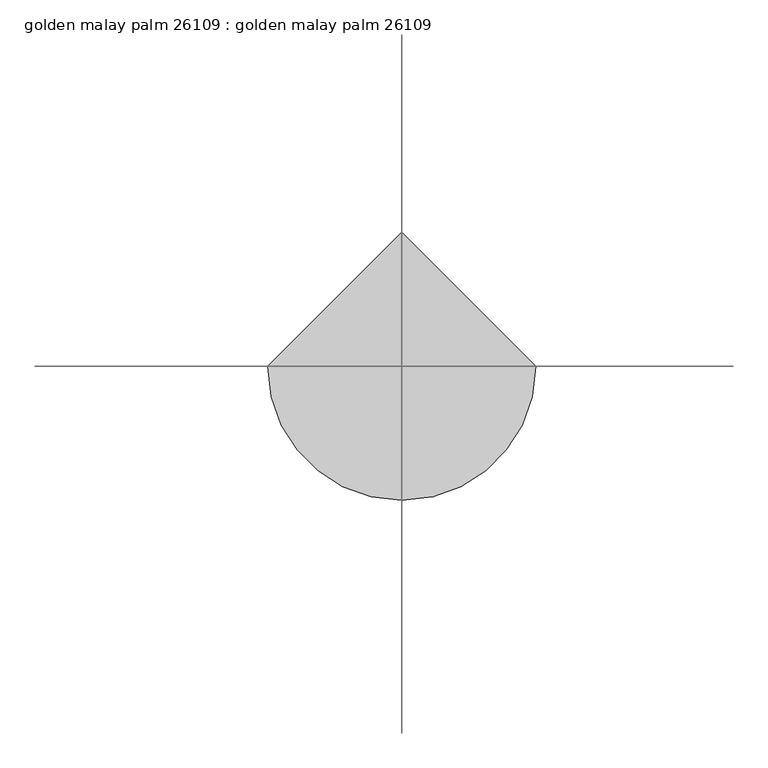
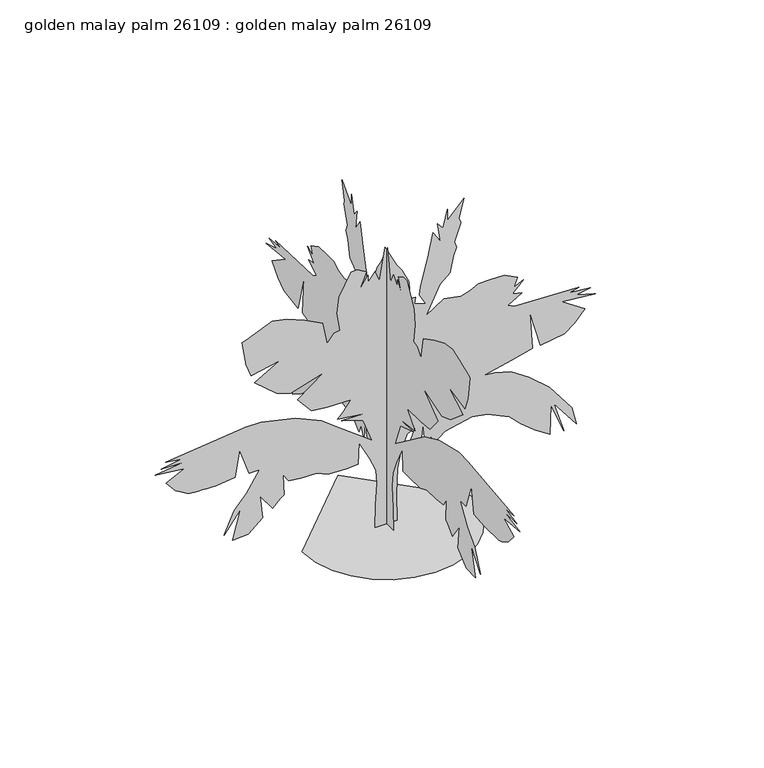
"""IFC4 building model written with IfcOpenShell, lengths in millimetres: proxy geometry, golden malay palm 26109 : golden malay palm 26109."""

from ifc_helpers import new_model, si_unit, origin, place, context, project, spatial, triangles, source, transform, mapped, element, save


def golden_malay_palm_26109_golden_malay_palm_26109_a310d7cf(model_context):
    return source(origin(), model_context, "Body", "Tessellation", [
        triangles([(9.89e-05, 133.5213922, 670.0644053), (0.0001158, 103.2936315, 529.0005229), (0.0001458, 93.2174569, 277.101182), (0.0001788, 98.2555397, 0.010878), (0.0001788, -113.3400931, 0.010878), (0.0001518, -108.30251, 226.7208087), (0.000126, -93.1884979, 443.3542972), (0.0001098, -103.2644181, 579.3813867), (9.23e-05, -163.7202029, 725.4820982), (6.95e-05, -264.479932, 916.9269533), (9.53e-05, -274.5561157, 700.292938), (9.59e-05, -385.3915197, 695.2536381), (9.53e-05, -561.7207641, 700.292938), (8.93e-05, -672.5587297, 750.671331), (8.93e-05, -828.7356068, 750.671331), (8.75e-05, -944.6103653, 765.7868328), (7.79e-05, -994.9887583, 846.3936859), (0.0001026, -984.9125565, 639.8358725), (0.0001056, -1025.2172184, 614.6467123), (0.0001146, -1095.7504858, 539.0766884), (9.47e-05, -1216.6620735, 705.3297672), (0.0001218, -1191.4703699, 478.6196228), (0.0001362, -1332.536832, 357.7080714), (0.0001368, -1483.6744091, 352.6712422), (0.0001026, -1403.067556, 639.8358725), (0.0001272, -1564.283733, 433.2780953), (0.000102, -1468.5613781, 644.8752451), (8.57e-05, -1347.6498631, 780.8998638), (6.23e-05, -1221.69883, 977.3814754), (6.23e-05, -1322.4607029, 977.3814754), (3.11e-05, -1413.1436852, 1239.3569092), (6.17e-05, -1458.4852489, 982.4207754), (6.41e-05, -1639.8538296, 962.2684444), (6.4e-05, -1687.1180958, 963.3555874), (6.38e-05, -1732.9753258, 964.4858963), (6.37e-05, -1776.0104897, 965.7050806), (6.35e-05, -1814.8165512, 967.0563789), (6.34e-05, -1847.9838581, 968.5828846), (6.32e-05, -1874.0976711, 970.3329231), (6.29e-05, -1891.7531342, 972.3446463), (6.24e-05, -1906.0304604, 976.2663546), (6.16e-05, -1922.6852577, 983.3606163), (6.04e-05, -1941.3262711, 993.0989754), (5.9e-05, -1961.5497459, 1004.9505775), (5.74e-05, -1982.9670433, 1018.3922716), (5.57e-05, -2005.1742634, 1032.8880438), (5.39e-05, -2027.7802963, 1047.9146702), (4.13e-05, -2118.4632786, 1153.7132269), (3.11e-05, -1947.1708271, 1239.3569092), (2.75e-05, -2224.261908, 1269.585442), (2.27e-05, -1952.2101997, 1309.8901039), (2.21e-05, -2168.844215, 1314.9270058), (1.79e-05, -1977.3993599, 1350.1949112), (1.55e-05, -2123.5001804, 1370.3471695), (5.3e-06, -1357.7259922, 1455.9909245), (5.3e-06, -1206.5858717, 1455.9909245), (1.43e-05, -874.0771706, 1380.4208279), (2.81e-05, -627.2171659, 1264.5486855), (4.37e-05, -455.9247508, 1133.5608959), (7.19e-05, -138.5302706, 896.7745497), (4.37e-05, -229.2143339, 1133.5608959), (3.59e-05, -435.7723835, 1199.0547907), (3.65e-05, -219.1381502, 1194.0154181), (3.23e-05, -471.0377455, 1229.2832508), (2.63e-05, -420.6568454, 1279.6617165), (1.43e-05, -340.0499923, 1380.4208279), (1.37e-05, -571.7995093, 1385.4602005), (1.19e-05, -722.9370501, 1400.5732315), (-7.4e-06, -858.9641396, 1561.7895538), (-2.96e-05, -607.064835, 1748.194891), (-1.82e-05, -924.4580343, 1652.4750069), (-2.36e-05, -1060.4851238, 1697.8165707), (-4.52e-05, -1272.0797665, 1879.1826805), (-6.14e-05, -1030.256591, 2015.2098427), (-5.48e-05, -1302.3082993, 1959.7921497), (-7.04e-05, -1352.6890903, 2090.7797939), (-9.86e-05, -1387.954525, 2327.5662128), (-9.98e-05, -1352.6890903, 2337.642342), (-0.000107, -1211.6227009, 2398.0967915), (-0.0001125, -1100.787315, 2443.4383553), (-0.0001095, -964.7627689, 2418.2491951), (-0.0001004, -788.4309448, 2342.6790985), (-8.96e-05, -617.1410368, 2251.9961163), (-6.32e-05, -571.7995093, 2030.3227283), (-7.28e-05, -506.3030711, 2110.9321976), (-7.4e-05, -445.848549, 2121.0083267), (-9.62e-05, -476.0770818, 2307.4138092), (-0.0001149, -455.9247508, 2463.5906136), (-0.0001401, -340.0499923, 2675.1776985), (-0.0001407, -284.6322812, 2680.2323318), (-0.0001347, -193.9479727, 2629.8386055), (-0.0001155, -259.443121, 2468.6301315), (-0.0001299, -178.834215, 2589.5288567), (-0.0001215, -178.834215, 2519.0084518), (-0.0001311, -113.3400931, 2599.6128342), (-0.0001185, -67.9985656, 2493.8192917), (-0.0001569, -17.6182708, 2816.2493202), (-0.0001311, 93.2174569, 2599.6128342), (-0.0001221, 148.6356586, 2524.0476791), (-0.0001052, 214.1292808, 2382.9839058), (-8.42e-05, 224.2057188, 2206.6545525), (-8.42e-05, 279.6234118, 2206.6545525), (-7.64e-05, 269.5472281, 2141.1607304), (-7.16e-05, 380.3826322, 2100.8560684), (-8.48e-05, 314.8887374, 2211.6914543), (-9.5e-05, 324.9649392, 2297.3376801), (-0.0001275, 395.4981703, 2569.3867722), (-0.0001551, 445.8764906, 2801.1362892), (-0.0001419, 516.4097217, 2690.2907295), (-0.0001641, 491.2205615, 2876.7011536), (-0.0001563, 541.5989182, 2811.219976), (-0.0001779, 586.9404093, 2992.5760574), (-0.0001641, 586.9404093, 2876.7011536), (-0.0001845, 743.1199024, 3047.9988373), (-0.0001623, 697.7783386, 2861.5881226), (-0.0001569, 712.8913696, 2816.2493202), (-0.0001359, 652.434304, 2639.922583), (-0.0001281, 672.586635, 2574.4158257), (-0.0001191, 642.3581022, 2498.8561935), (-9.98e-05, 607.0927766, 2337.642342), (-9.02e-05, 511.3703854, 2257.0328728), (-5.72e-05, 380.3826322, 1979.944408), (-7.1e-05, 551.6750836, 2095.8166958), (-6.68e-05, 712.8913696, 2060.5512611), (-6.98e-05, 803.5744246, 2085.7404213), (-7.52e-05, 884.1838211, 2131.0846012), (-7.52e-05, 995.019207, 2131.0846012), (-7.52e-05, 1131.0462965, 2131.0846012), (-6.74e-05, 1256.9946407, 2065.5906338), (-5.66e-05, 1226.7661079, 1974.9050354), (-6.2e-05, 1317.4517063, 2020.2465992), (-4.94e-05, 1211.6531496, 1914.4505859), (-4.7e-05, 1302.3362045, 1894.2981823), (-3.74e-05, 1166.3116585, 1813.6888584), (-3.32e-05, 1231.8054806, 1778.4234238), (-3.02e-05, 1851.4788483, 1753.2342636), (-2.78e-05, 1755.7564934, 1733.0820053), (-2.54e-05, 1962.3143795, 1712.9296017), (-2.24e-05, 1826.2896881, 1687.7404415), (-1.58e-05, 2007.655798, 1632.3227486), (-2e-05, 1685.2257694, 1667.5880379), (-1.9e-06, 1906.8966866, 1516.44799), (1.13e-05, 1806.1374298, 1405.6126041), (2.03e-05, 1710.4149296, 1330.0425076), (2.45e-05, 1478.6680286, 1294.7772182), (-1.94e-05, 1377.9063011, 1662.5486652), (2.45e-05, 1403.0979321, 1294.7772182), (3.05e-05, 1211.6531496, 1244.3962818), (3.77e-05, 934.5621414, 1183.9392162), (3.95e-05, 1040.3606981, 1168.8262579), (4.43e-05, 1196.5401913, 1128.5215233), (5.81e-05, 1367.8300266, 1012.6493082), (7.85e-05, 1564.3117836, 841.3568567), (0.0001128, 1780.9482697, 554.1896831), (0.0001338, 1826.2896881, 377.8604024), (0.0001007, 1609.6558182, 654.9514469), (0.0001374, 1705.3781731, 347.6318696), (0.0001014, 1579.4272854, 649.9120743), (0.0001356, 1569.3510109, 362.7474077), (0.0001242, 1423.2503357, 458.4697989), (0.0001116, 1292.2600754, 564.2658485), (9.83e-05, 1181.4246168, 675.1012344), (8.63e-05, 969.8300468, 775.8630346), (8.33e-05, 818.6899263, 801.0521948), (8.99e-05, 561.7512491, 745.6345018), (0.0001001, 455.9526924, 659.9882761), (9.05e-05, 425.7267031, 740.5976727), (0.0001032, 380.3826322, 634.7991159), (7.43e-05, 350.1566428, 876.6222187), (9.71e-05, 324.9649392, 685.1774363), (9.89e-05, 234.2813756, 670.0644053), (8.63e-05, 234.2813756, 775.8630346), (7.31e-05, 279.6234118, 886.6984205), (7.85e-05, 193.9774404, 841.3568567), (8.87e-05, 163.7496706, 755.710631), (133.5213922, 0.0001645, 670.0644053), (103.2936315, 0.0001813, 529.0005229), (93.2174569, 0.0002114, 277.101182), (98.2555397, 0.0002444, 0.0107758), (-113.3400931, 0.0002444, 0.0108645), (-108.30251, 0.0002174, 226.7208087), (-93.1887523, 0.0001915, 443.3542972), (-103.2644181, 0.0001753, 579.3813867), (-163.7204573, 0.0001579, 725.4820982), (-264.479932, 0.0001351, 916.9269533), (-274.5561157, 0.0001609, 700.292938), (-385.3915197, 0.0001615, 695.2536381), (-561.7233075, 0.0001609, 700.292938), (-672.5587297, 0.0001549, 750.671331), (-828.7356068, 0.0001549, 750.671331), (-944.6103653, 0.0001531, 765.7868328), (-994.9912291, 0.0001435, 846.3936859), (-984.9125565, 0.0001681, 639.8358725), (-1025.2172184, 0.0001711, 614.6467123), (-1095.7504858, 0.0001801, 539.0766884), (-1216.6620735, 0.0001603, 705.3297672), (-1191.4703699, 0.0001873, 478.6196228), (-1332.536832, 0.0002018, 357.7080714), (-1483.6744091, 0.0002024, 352.6712422), (-1403.067556, 0.0001681, 639.8358725), (-1564.283733, 0.0001927, 433.2780953), (-1468.5613781, 0.0001675, 644.8752451), (-1347.6498631, 0.0001513, 780.8998638), (-1221.69883, 0.0001279, 977.3814754), (-1322.4607029, 0.0001279, 977.3814754), (-1413.1436852, 9.67e-05, 1239.3569092), (-1458.4852489, 0.0001273, 982.4207754), (-1639.8538296, 0.0001297, 962.2684444), (-1687.1180958, 0.0001296, 963.3555874), (-1732.9753258, 0.0001294, 964.4858963), (-1776.0104897, 0.0001293, 965.7050806), (-1814.8165512, 0.0001291, 967.0563789), (-1847.9838581, 0.0001289, 968.5828846), (-1874.0976711, 0.0001287, 970.3329231), (-1891.7531342, 0.0001285, 972.3446463), (-1906.0304604, 0.000128, 976.2663546), (-1922.6852577, 0.0001272, 983.3606163), (-1941.3262711, 0.000126, 993.0989754), (-1961.5497459, 0.0001246, 1004.9505775), (-1982.9670433, 0.000123, 1018.3922716), (-2005.1742634, 0.0001213, 1032.8880438), (-2027.7802963, 0.0001195, 1047.9146702), (-2118.4632786, 0.0001069, 1153.7132269), (-1947.1708271, 9.67e-05, 1239.3569092), (-2224.261908, 9.31e-05, 1269.585442), (-1952.2101997, 8.82e-05, 1309.8901039), (-2168.844215, 8.76e-05, 1314.9270058), (-1977.3993599, 8.34e-05, 1350.1949112), (-2123.5001804, 8.1e-05, 1370.3471695), (-1357.7259922, 7.08e-05, 1455.9909245), (-1206.5858717, 7.08e-05, 1455.9909245), (-874.0771706, 7.98e-05, 1380.4208279), (-627.2171659, 9.37e-05, 1264.5486855), (-455.9247508, 0.0001093, 1133.5608959), (-138.5302706, 0.0001375, 896.7745497), (-229.2145882, 0.0001093, 1133.5608959), (-435.7723835, 0.0001015, 1199.0547907), (-219.1381502, 0.0001021, 1194.0154181), (-471.0377455, 9.79e-05, 1229.2832508), (-420.6593888, 9.18e-05, 1279.6617165), (-340.0499923, 7.98e-05, 1380.4208279), (-571.7995093, 7.92e-05, 1385.4602005), (-722.9370501, 7.74e-05, 1400.5732315), (-858.9641396, 5.82e-05, 1561.7895538), (-607.064835, 3.6e-05, 1748.194891), (-924.4580343, 4.74e-05, 1652.4750069), (-1060.4851238, 4.2e-05, 1697.8165707), (-1272.0797665, 2.04e-05, 1879.1826805), (-1030.256591, 4.2e-06, 2015.2098427), (-1302.3082993, 1.08e-05, 1959.7921497), (-1352.6890903, -4.8e-06, 2090.7797939), (-1387.954525, -3.31e-05, 2327.5662128), (-1352.6890903, -3.43e-05, 2337.642342), (-1211.6227009, -4.15e-05, 2398.0967915), (-1100.787315, -4.69e-05, 2443.4383553), (-964.7627689, -4.39e-05, 2418.2491951), (-788.4309448, -3.49e-05, 2342.6790985), (-617.1410368, -2.41e-05, 2251.9961163), (-571.7995093, 2.4e-06, 2030.3227283), (-506.3030711, -7.2e-06, 2110.9321976), (-445.848549, -8.4e-06, 2121.0083267), (-476.0770818, -3.07e-05, 2307.4138092), (-455.9247508, -4.93e-05, 2463.5906136), (-340.0499923, -7.45e-05, 2675.1776985), (-284.6322812, -7.51e-05, 2680.2323318), (-193.948227, -6.91e-05, 2629.8386055), (-259.443121, -4.99e-05, 2468.6301315), (-178.834215, -6.43e-05, 2589.5288567), (-178.834215, -5.59e-05, 2519.0084518), (-113.3400931, -6.55e-05, 2599.6128342), (-67.9985656, -5.29e-05, 2493.8192917), (-17.6183468, -9.13e-05, 2816.2493202), (93.2174569, -6.55e-05, 2599.6128342), (148.6356586, -5.65e-05, 2524.0476791), (214.1292808, -3.97e-05, 2382.9839058), (224.2054645, -1.87e-05, 2206.6545525), (279.6234118, -1.87e-05, 2206.6545525), (269.5472281, -1.08e-05, 2141.1607304), (380.3826322, -6e-06, 2100.8560684), (314.8887374, -1.93e-05, 2211.6914543), (324.9649392, -2.95e-05, 2297.3376801), (395.4981703, -6.19e-05, 2569.3867722), (445.8764906, -8.95e-05, 2801.1362892), (516.4097217, -7.63e-05, 2690.2907295), (491.2205615, -9.85e-05, 2876.7011536), (541.5989182, -9.07e-05, 2811.219976), (586.9404093, -0.0001123, 2992.5760574), (586.9404093, -9.85e-05, 2876.7011536), (743.1199024, -0.000119, 3047.9988373), (697.7757952, -9.67e-05, 2861.5881226), (712.8913696, -9.13e-05, 2816.2493202), (652.434304, -7.03e-05, 2639.922583), (672.586635, -6.25e-05, 2574.4158257), (642.3581022, -5.35e-05, 2498.8561935), (607.0927766, -3.43e-05, 2337.642342), (511.3703854, -2.47e-05, 2257.0328728), (380.3826322, 8.4e-06, 1979.944408), (551.6750836, -5.4e-06, 2095.8166958), (712.8913696, -1.2e-06, 2060.5512611), (803.5744246, -4.2e-06, 2085.7404213), (884.1838211, -9.6e-06, 2131.0846012), (995.019207, -9.6e-06, 2131.0846012), (1131.0462965, -9.6e-06, 2131.0846012), (1256.9946407, -1.8e-06, 2065.5906338), (1226.7661079, 9e-06, 1974.9050354), (1317.4517063, 3.6e-06, 2020.2465992), (1211.6531496, 1.62e-05, 1914.4505859), (1302.3362045, 1.86e-05, 1894.2981823), (1166.3116585, 2.82e-05, 1813.6888584), (1231.8054806, 3.24e-05, 1778.4234238), (1851.4788483, 3.54e-05, 1753.2342636), (1755.7564934, 3.78e-05, 1733.0820053), (1962.3143795, 4.02e-05, 1712.9296017), (1826.2896881, 4.32e-05, 1687.7404415), (2007.655798, 4.98e-05, 1632.3227486), (1685.2232986, 4.56e-05, 1667.5880379), (1906.8966866, 6.36e-05, 1516.44799), (1806.1374298, 7.68e-05, 1405.6126041), (1710.4149296, 8.58e-05, 1330.0425076), (1478.6680286, 9e-05, 1294.7772182), (1377.9063011, 4.62e-05, 1662.5486652), (1403.0954613, 9e-05, 1294.7772182), (1211.6531496, 9.61e-05, 1244.3962818), (934.5621414, 0.0001033, 1183.9392162), (1040.3606981, 0.0001051, 1168.8262579), (1196.5401913, 0.0001099, 1128.5215233), (1367.8300266, 0.0001237, 1012.6493082), (1564.3117836, 0.0001441, 841.3568567), (1780.9456535, 0.0001783, 554.1896831), (1826.2896881, 0.0001994, 377.8604024), (1609.6558182, 0.0001663, 654.9514469), (1705.3757023, 0.000203, 347.6318696), (1579.4272854, 0.0001669, 649.9120743), (1569.3510109, 0.0002012, 362.7474077), (1423.2503357, 0.0001897, 458.4672918), (1292.2600754, 0.0001771, 564.2658485), (1181.4246168, 0.0001639, 675.1012344), (969.8300468, 0.0001519, 775.8630346), (818.6899263, 0.0001489, 801.0521948), (561.7512491, 0.0001555, 745.6345018), (455.9526924, 0.0001657, 659.9882761), (425.7241596, 0.0001561, 740.5951292), (380.3826322, 0.0001687, 634.7991159), (350.1566428, 0.0001399, 876.6222187), (324.9649392, 0.0001627, 685.1774363), (234.2813756, 0.0001645, 670.0644053), (234.2813756, 0.0001519, 775.8630346), (279.6234118, 0.0001387, 886.6984205), (193.9774404, 0.0001441, 841.3568567), (163.7496706, 0.0001543, 755.710631), (-812.451717, 0.0, 7.05e-05), (-790.9734495, -186.160076, 7.3e-05), (-729.802692, -357.1187905, 8.03e-05), (-633.8364567, -507.9769515, 9.18e-05), (-507.9769515, -633.8364567, 0.0001068), (-357.1187905, -729.802692, 1.08e-05), (-186.1598216, -790.9734495, 3.12e-05), (3.55e-05, -812.451717, 5.34e-05), (186.160076, -790.9734495, 7.56e-05), (357.1187905, -729.802692, 9.6e-05), (507.9769515, -633.8364567, 0.0), (633.8364567, -507.9769515, 1.5e-05), (729.802692, -357.1187905, 2.64e-05), (790.9734495, -186.1598216, 3.37e-05), (812.451717, 7.1e-05, 3.63e-05), (-0.0001065, 812.451717, 5.34e-05)], [[157, 156, 158], [140, 139, 141], [52, 51, 53], [26, 25, 27], [112, 111, 113], [136, 135, 137], [54, 53, 55], [50, 49, 51], [138, 137, 139], [62, 61, 63], [131, 130, 132], [155, 154, 156], [154, 153, 156], [114, 113, 115], [110, 109, 111], [168, 167, 169], [93, 92, 94], [97, 96, 98], [139, 137, 141], [133, 132, 134], [108, 107, 109], [137, 135, 141], [27, 25, 28], [64, 63, 65], [159, 158, 160], [95, 94, 96], [53, 51, 55], [73, 72, 74], [166, 165, 167], [24, 23, 25], [23, 22, 25], [22, 21, 25], [25, 21, 28], [65, 63, 66], [48, 47, 49], [20, 19, 21], [171, 170, 172], [170, 169, 172], [172, 169, 173], [102, 101, 103], [142, 141, 143], [156, 153, 158], [69, 68, 70], [68, 67, 70], [28, 21, 29], [5, 4, 6], [4, 3, 6], [6, 3, 7], [3, 2, 7], [7, 2, 8], [2, 1, 8], [160, 158, 161], [8, 1, 9], [98, 96, 99], [11, 10, 12], [145, 144, 146], [144, 143, 146], [143, 141, 146], [141, 135, 146], [67, 66, 70], [91, 90, 92], [90, 89, 92], [89, 88, 92], [77, 76, 78], [88, 87, 92], [1, 175, 9], [129, 128, 130], [75, 74, 76], [51, 49, 55], [47, 46, 49], [147, 146, 148], [158, 153, 161], [153, 152, 161], [161, 152, 162], [162, 152, 163], [152, 151, 163], [151, 150, 163], [150, 149, 163], [163, 149, 164], [72, 71, 74], [71, 70, 74], [76, 74, 78], [78, 74, 79], [79, 74, 80], [80, 74, 81], [81, 74, 82], [74, 70, 82], [82, 70, 83], [83, 70, 84], [32, 31, 33], [146, 135, 148], [148, 135, 149], [135, 134, 149], [99, 96, 100], [46, 45, 49], [30, 29, 31], [9, 175, 10], [175, 174, 10], [45, 44, 49], [49, 44, 55], [44, 43, 55], [43, 42, 55], [42, 41, 55], [41, 40, 55], [40, 39, 55], [39, 38, 55], [38, 37, 55], [37, 36, 55], [36, 35, 55], [35, 34, 55], [34, 33, 55], [33, 31, 55], [55, 31, 56], [31, 29, 56], [56, 29, 57], [57, 29, 58], [100, 96, 101], [29, 21, 58], [115, 113, 116], [116, 113, 117], [113, 111, 117], [111, 109, 117], [109, 107, 117], [117, 107, 118], [118, 107, 119], [107, 106, 119], [119, 106, 120], [120, 106, 121], [106, 105, 121], [105, 104, 121], [121, 104, 122], [104, 103, 122], [167, 165, 169], [12, 10, 13], [87, 86, 92], [164, 149, 165], [165, 149, 169], [18, 17, 19], [19, 17, 21], [21, 17, 58], [58, 17, 59], [17, 16, 59], [16, 15, 59], [15, 14, 59], [14, 13, 59], [13, 10, 59], [59, 10, 60], [10, 174, 60], [60, 174, 61], [61, 174, 63], [174, 173, 63], [128, 127, 130], [130, 127, 132], [132, 127, 134], [127, 126, 134], [126, 125, 134], [134, 125, 149], [125, 124, 149], [149, 124, 169], [124, 123, 169], [123, 122, 169], [169, 122, 173], [173, 122, 63], [63, 122, 66], [66, 122, 70], [122, 103, 70], [70, 103, 84], [84, 103, 85], [85, 103, 86], [103, 101, 86], [101, 96, 86], [86, 96, 92], [96, 94, 92], [331, 332, 333], [314, 315, 316], [226, 227, 228], [200, 201, 202], [286, 287, 288], [310, 311, 312], [228, 229, 230], [224, 225, 226], [312, 313, 314], [236, 237, 238], [305, 306, 307], [329, 330, 331], [328, 329, 331], [288, 289, 290], [284, 285, 286], [342, 343, 344], [267, 268, 269], [271, 272, 273], [312, 314, 316], [307, 308, 309], [282, 283, 284], [310, 312, 316], [200, 202, 203], [238, 239, 240], [333, 334, 335], [269, 270, 271], [226, 228, 230], [247, 248, 249], [340, 341, 342], [198, 199, 200], [197, 198, 200], [196, 197, 200], [196, 200, 203], [238, 240, 241], [222, 223, 224], [194, 195, 196], [345, 346, 347], [344, 345, 347], [344, 347, 348], [276, 277, 278], [316, 317, 318], [328, 331, 333], [243, 244, 245], [242, 243, 245], [196, 203, 204], [179, 180, 181], [178, 179, 181], [178, 181, 182], [177, 178, 182], [177, 182, 183], [176, 177, 183], [333, 335, 336], [176, 183, 184], [271, 273, 274], [185, 186, 187], [319, 320, 321], [318, 319, 321], [316, 318, 321], [310, 316, 321], [241, 242, 245], [265, 266, 267], [264, 265, 267], [263, 264, 267], [251, 252, 253], [262, 263, 267], [350, 176, 184], [303, 304, 305], [249, 250, 251], [224, 226, 230], [221, 222, 224], [321, 322, 323], [328, 333, 336], [327, 328, 336], [327, 336, 337], [327, 337, 338], [326, 327, 338], [325, 326, 338], [324, 325, 338], [324, 338, 339], [246, 247, 249], [245, 246, 249], [249, 251, 253], [249, 253, 254], [249, 254, 255], [249, 255, 256], [249, 256, 257], [245, 249, 257], [245, 257, 258], [245, 258, 259], [206, 207, 208], [310, 321, 323], [310, 323, 324], [309, 310, 324], [271, 274, 275], [220, 221, 224], [204, 205, 206], [350, 184, 185], [349, 350, 185], [219, 220, 224], [219, 224, 230], [218, 219, 230], [217, 218, 230], [216, 217, 230], [215, 216, 230], [214, 215, 230], [213, 214, 230], [212, 213, 230], [211, 212, 230], [210, 211, 230], [209, 210, 230], [208, 209, 230], [206, 208, 230], [206, 230, 231], [204, 206, 231], [204, 231, 232], [204, 232, 233], [271, 275, 276], [196, 204, 233], [288, 290, 291], [288, 291, 292], [286, 288, 292], [284, 286, 292], [282, 284, 292], [282, 292, 293], [282, 293, 294], [281, 282, 294], [281, 294, 295], [281, 295, 296], [280, 281, 296], [279, 280, 296], [279, 296, 297], [278, 279, 297], [340, 342, 344], [185, 187, 188], [261, 262, 267], [324, 339, 340], [324, 340, 344], [192, 193, 194], [192, 194, 196], [192, 196, 233], [192, 233, 234], [191, 192, 234], [190, 191, 234], [189, 190, 234], [188, 189, 234], [185, 188, 234], [185, 234, 235], [349, 185, 235], [349, 235, 236], [349, 236, 238], [348, 349, 238], [302, 303, 305], [302, 305, 307], [302, 307, 309], [301, 302, 309], [300, 301, 309], [300, 309, 324], [299, 300, 324], [299, 324, 344], [298, 299, 344], [297, 298, 344], [297, 344, 348], [297, 348, 238], [297, 238, 241], [297, 241, 245], [278, 297, 245], [278, 245, 259], [278, 259, 260], [278, 260, 261], [276, 278, 261], [271, 276, 261], [271, 261, 267], [269, 271, 267], [365, 366, 351], [364, 365, 351], [364, 351, 352], [363, 364, 352], [363, 352, 353], [363, 353, 354], [362, 363, 354], [361, 362, 354], [361, 354, 355], [361, 355, 356], [361, 356, 357], [361, 357, 358], [361, 358, 359], [361, 359, 360]], closed=False),
    ])


if __name__ == "__main__":
    model = new_model("IFC4")
    model_context = context("Model", 3, world=origin())
    ifc_project = project(units=[si_unit("LENGTHUNIT", "METRE", prefix="MILLI")], contexts=[model_context])
    site = spatial("IfcSite", under=ifc_project)
    building = spatial("IfcBuilding", under=site)
    placement = place(None, origin())
    golden_malay_palm_26109_golden_malay_palm_26109_shape = golden_malay_palm_26109_golden_malay_palm_26109_a310d7cf(model_context)
    element("IfcBuildingElementProxy", 1, Name="golden malay palm 26109 : golden malay palm 26109", ObjectType="golden malay palm 26109 : golden malay palm 26109", at=placement, inside=building, context=model_context, shape_type="MappedRepresentation", body=[
        mapped(golden_malay_palm_26109_golden_malay_palm_26109_shape, transform((0.0, 0.0, 0.0), x_axis=(1.0, 0.0, 0.0), y_axis=(0.0, 1.0, 0.0), z_axis=(0.0, 0.0, 1.0))),
    ])
    save(model, "model.ifc")

# Revit data of these elements
# Type "golden malay palm 26109 : golden malay palm 26109"
#   built-in parameter 1005195 = "RPC-16-FXGM-2RXX-PGXL-E000-ST1L-LVER-AU"
#   Height = 0
